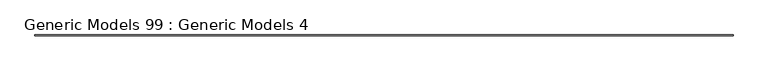
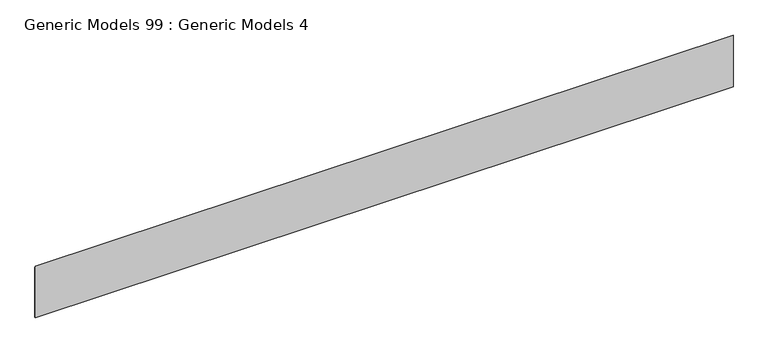
"""IFC4 building model written with IfcOpenShell, lengths in millimetres: proxy geometry, Generic Models 99 : Generic Models 4."""

import ifcopenshell
import ifcopenshell.guid

model = None  # the IFC model being written
_history = None  # IfcOwnerHistory: only IFC2X3 demands one
_inside = {}  # id of a spatial element -> (the spatial element, [elements in it])
_under = {}  # id of a project, library or spatial element -> (it, [spatial elements below it])
_declared = {}  # id of a project -> (the project, [libraries it declares])
_typed = {}  # id of a type object -> (the type object, [elements of that type])
_made_of = {}  # id of a material, layer set ... -> (it, [elements and type objects made of it])


def new_model(schema):
    """Start an empty IFC model of exactly this schema.

    Asked for "IFC4X3", IfcOpenShell would pick the latest addendum, in which some entities
    have other attributes; the version numbers below select the first issue.
    IFC2X3 requires an IfcOwnerHistory on every rooted entity: one is made here for all.
    """
    global model, _history
    if schema == "IFC4X3":
        model = ifcopenshell.file(schema_version=(4, 3, 0, 0))
    else:
        model = ifcopenshell.file(schema=schema)
    _inside.clear()
    _under.clear()
    _declared.clear()
    _typed.clear()
    _made_of.clear()
    _history = None
    if model.schema == "IFC2X3":
        org = make("IfcOrganization", Name="unknown")
        user = make(
            "IfcPersonAndOrganization",
            ThePerson=make("IfcPerson", FamilyName="unknown"),
            TheOrganization=org,
        )
        app = make(
            "IfcApplication",
            ApplicationDeveloper=org,
            Version="unknown",
            ApplicationFullName="unknown",
            ApplicationIdentifier="unknown",
        )
        _history = make(
            "IfcOwnerHistory",
            OwningUser=user,
            OwningApplication=app,
            ChangeAction="ADDED",
            CreationDate=0,
        )
    return model


def make(cls, **values):
    """One entity of the class cls with the attributes given. An attribute that is None is left unset."""
    return model.create_entity(
        cls, **{name: value for name, value in values.items() if value is not None}
    )


def rooted(cls, **values):
    """An entity with a GlobalId (a new one), such as an element, a storey or a relation."""
    return make(cls, GlobalId=ifcopenshell.guid.new(), OwnerHistory=_history, **values)


def si_unit(unit_type, name, prefix=None):
    """IfcSIUnit, for example si_unit("LENGTHUNIT", "METRE", prefix="MILLI")."""
    return make("IfcSIUnit", UnitType=unit_type, Prefix=prefix, Name=name)


def assignment(units):
    """IfcUnitAssignment: the units of a project."""
    return None if units is None else make("IfcUnitAssignment", Units=units)


def point(xyz):
    """IfcCartesianPoint."""
    return None if xyz is None else make("IfcCartesianPoint", Coordinates=xyz)


def direction(xyz):
    """IfcDirection."""
    return None if xyz is None else make("IfcDirection", DirectionRatios=xyz)


def frame(location, z_axis=None, x_axis=None):
    """IfcAxis2Placement3D, a coordinate frame: its origin and axes. An axis left out is left unset."""
    return make(
        "IfcAxis2Placement3D",
        Location=point(location),
        Axis=direction(z_axis),
        RefDirection=direction(x_axis),
    )


def origin():
    """The frame at (0, 0, 0) with its axes left unset."""
    return frame((0.0, 0.0, 0.0))


def place(relative_to, where):
    """IfcLocalPlacement: puts the frame where relative to a parent placement (None: the world)."""
    return make(
        "IfcLocalPlacement", PlacementRelTo=relative_to, RelativePlacement=where
    )


def context(
    kind, dimensions, precision=None, world=None, true_north=None, identifier=None
):
    """IfcGeometricRepresentationContext, for example the 3D "Model" context."""
    return make(
        "IfcGeometricRepresentationContext",
        ContextIdentifier=identifier,
        ContextType=kind,
        CoordinateSpaceDimension=dimensions,
        Precision=precision,
        WorldCoordinateSystem=world,
        TrueNorth=true_north,
    )


def project(units=None, contexts=None):
    """IfcProject with its units and contexts."""
    return rooted(
        "IfcProject",
        Name="project",
        RepresentationContexts=contexts,
        UnitsInContext=assignment(units),
    )


def spatial(cls, under=None, at=None, **own):
    """A site, building, storey or space (cls), placed at a placement, below another one or the project."""
    s = rooted(cls, ObjectPlacement=at, **own)
    if under is not None:
        _under.setdefault(under.id(), (under, []))[1].append(s)
    return s


def polyline(points):
    """IfcPolyline through the points."""
    return make("IfcPolyline", Points=[point(p) for p in points])


def outline(outer, holes=None, kind="AREA"):
    """IfcArbitraryClosedProfileDef: a profile drawn as a closed curve; with holes, ...WithVoids."""
    if holes is None:
        return make("IfcArbitraryClosedProfileDef", ProfileType=kind, OuterCurve=outer)
    return make(
        "IfcArbitraryProfileDefWithVoids",
        ProfileType=kind,
        OuterCurve=outer,
        InnerCurves=holes,
    )


def extrude(swept, where, along, depth):
    """IfcExtrudedAreaSolid: the profile swept, set in the frame where, extruded along a direction by depth."""
    return make(
        "IfcExtrudedAreaSolid",
        SweptArea=swept,
        Position=where,
        ExtrudedDirection=direction(along),
        Depth=depth,
    )


def shape(context_of_items, identifier, shape_type, items):
    """IfcShapeRepresentation: the items that make up one representation, for example the "Body"."""
    return make(
        "IfcShapeRepresentation",
        ContextOfItems=context_of_items,
        RepresentationIdentifier=identifier,
        RepresentationType=shape_type,
        Items=items,
    )


def source(mapping_origin, context_of_items, identifier, shape_type, items):
    """IfcRepresentationMap: a shape defined once, which mapped items show again and again."""
    return make(
        "IfcRepresentationMap",
        MappingOrigin=mapping_origin,
        MappedRepresentation=shape(context_of_items, identifier, shape_type, items),
    )


def transform(
    local_origin,
    x_axis=None,
    y_axis=None,
    z_axis=None,
    scale=None,
    scale2=None,
    scale3=None,
    uniform=True,
):
    """IfcCartesianTransformationOperator3D, or its non-uniform kind. x_axis, y_axis, z_axis: its Axis1, 2, 3."""
    if uniform:
        return make(
            "IfcCartesianTransformationOperator3D",
            Axis1=direction(x_axis),
            Axis2=direction(y_axis),
            LocalOrigin=point(local_origin),
            Scale=scale,
            Axis3=direction(z_axis),
        )
    return make(
        "IfcCartesianTransformationOperator3DnonUniform",
        Axis1=direction(x_axis),
        Axis2=direction(y_axis),
        LocalOrigin=point(local_origin),
        Scale=scale,
        Axis3=direction(z_axis),
        Scale2=scale2,
        Scale3=scale3,
    )


def mapped(mapping_source, mapping_target):
    """IfcMappedItem: shows the shape of a source again, moved by a transform."""
    return make(
        "IfcMappedItem", MappingSource=mapping_source, MappingTarget=mapping_target
    )


def made_of(thing, what):
    """Note that an element or type object is made of a material, layer set ...; save() writes the relation."""
    if what is not None:
        _made_of.setdefault(what.id(), (what, []))[1].append(thing)
    return thing


def element(
    cls,
    number,
    at=None,
    inside=None,
    cuts=None,
    type_object=None,
    material=None,
    context=None,
    identifier="Body",
    shape_type=None,
    held_by="IfcProductDefinitionShape",
    body=None,
    shapes=None,
    **own,
):
    """One element of the class cls, such as IfcWall. Its Tag is "e" and its number.

    at: its placement. inside: the storey or other place that contains it. cuts: it is an
    opening in that element (IfcRelVoidsElement). A single representation is given by context,
    identifier, shape_type and body (its items); several are given by shapes. held_by: the class
    of the entity that holds the representations. save() writes the other relations.
    """
    e = rooted(cls, Tag="e%d" % number, ObjectPlacement=at, **own)
    if body is not None:
        shapes = [shape(context, identifier, shape_type, body)]
    if shapes is not None:
        e.Representation = make(held_by, Representations=shapes)
    if inside is not None:
        _inside.setdefault(inside.id(), (inside, []))[1].append(e)
    if cuts is not None:
        rooted(
            "IfcRelVoidsElement", RelatingBuildingElement=cuts, RelatedOpeningElement=e
        )
    if type_object is not None:
        _typed.setdefault(type_object.id(), (type_object, []))[1].append(e)
    return made_of(e, material)


def aggregate(whole, parts):
    """IfcRelAggregates: a whole, such as a stair, and the parts it consists of."""
    return rooted("IfcRelAggregates", RelatingObject=whole, RelatedObjects=parts)


def save(model, path):
    """Write the relations noted so far, then the file.

    IfcRelAggregates (storeys below a building ...), IfcRelContainedInSpatialStructure (elements
    in a storey), IfcRelDefinesByType, IfcRelAssociatesMaterial and IfcRelDeclares: one each for
    every whole, place, type object, material and project.
    """
    for whole, parts in _under.values():
        aggregate(whole, parts)
    for where, things in _inside.values():
        rooted(
            "IfcRelContainedInSpatialStructure",
            RelatedElements=things,
            RelatingStructure=where,
        )
    for kind, things in _typed.values():
        rooted("IfcRelDefinesByType", RelatedObjects=things, RelatingType=kind)
    for what, things in _made_of.values():
        rooted("IfcRelAssociatesMaterial", RelatedObjects=things, RelatingMaterial=what)
    for by, libraries in _declared.values():
        rooted("IfcRelDeclares", RelatingContext=by, RelatedDefinitions=libraries)
    model.write(path)


def generic_models_99_generic_models_4_d8dff29c(model_context):
    return source(origin(), model_context, "Body", "SweptSolid", [
        extrude(outline(polyline([(51291.6637962, 127106.7707574), (51291.6637962, 125692.9395983), (51272.5226718, 125692.9395983), (51272.5226718, 127144.0455785), (51291.6637962, 127106.7707574)])), frame((-20795.7733045, 0.0, 0.0), z_axis=(1.0, 0.0, 0.0), x_axis=(0.0, 1.0, 0.0)), (0.0, 0.0, 1.0), 18643.6),
    ])


if __name__ == "__main__":
    model = new_model("IFC4")
    model_context = context("Model", 3, world=origin())
    ifc_project = project(units=[si_unit("LENGTHUNIT", "METRE", prefix="MILLI")], contexts=[model_context])
    site = spatial("IfcSite", under=ifc_project)
    building = spatial("IfcBuilding", under=site)
    placement = place(None, origin())
    generic_models_99_generic_models_4_shape = generic_models_99_generic_models_4_d8dff29c(model_context)
    element("IfcBuildingElementProxy", 1, Name="Generic Models 99 : Generic Models 4", ObjectType="Generic Models 99 : Generic Models 4", at=placement, inside=building, context=model_context, shape_type="MappedRepresentation", body=[
        mapped(generic_models_99_generic_models_4_shape, transform((0.0, 0.0, 0.0), x_axis=(1.0, 0.0, 0.0), y_axis=(0.0, 1.0, 0.0), z_axis=(0.0, 0.0, 1.0))),
    ])
    save(model, "model.ifc")

# Revit data of these elements
# Element 1 (IfcBuildingElementProxy, "Generic Models 99 : Generic Models 4")
#   Materials on its faces: "_7/8\" SMOOTH TROWEL EXTERIOR STUCCO (COLOR PER OWNER)"
# Materials
#   "_7/8\" SMOOTH TROWEL EXTERIOR STUCCO (COLOR PER OWNER)": class "Generic", colour RGB 233 233 233, transparency 0, Cost = 0
